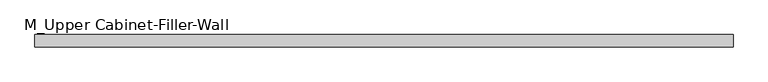
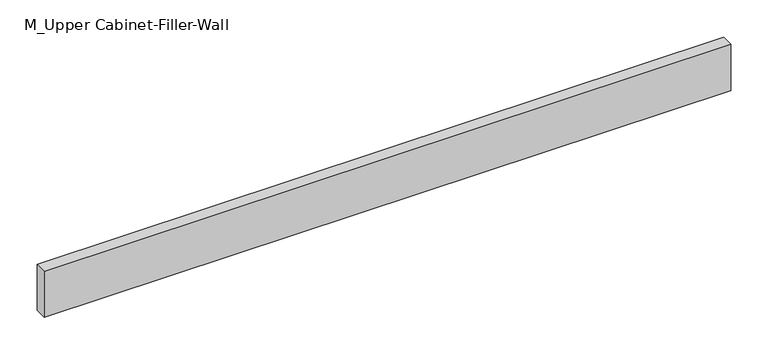
"""IFC4 building model written with IfcOpenShell, lengths in millimetres: furniture geometry, M_Upper Cabinet-Filler-Wall : fhorizontal2."""

from ifc_helpers import new_model, si_unit, frame, origin, place, context, project, spatial, polyline, outline, extrude, source, transform, mapped, element, save


def m_upper_cabinet_filler_wall_ea785238(model_context):
    return source(origin(), model_context, "Body", "SweptSolid", [
        extrude(outline(polyline([(-503.6288372, 38.1), (-503.6288372, 57.15), (563.1711628, 57.15), (563.1711628, 38.1), (-503.6288372, 38.1)])), frame((0.0, 0.0, 1923.8), z_axis=(0.0, 0.0, 1.0), x_axis=(1.0, 0.0, 0.0)), (0.0, 0.0, 1.0), 76.2),
    ])


if __name__ == "__main__":
    model = new_model("IFC4")
    model_context = context("Model", 3, world=origin())
    ifc_project = project(units=[si_unit("LENGTHUNIT", "METRE", prefix="MILLI")], contexts=[model_context])
    site = spatial("IfcSite", under=ifc_project)
    building = spatial("IfcBuilding", under=site)
    placement = place(None, origin())
    m_upper_cabinet_filler_wall_shape = m_upper_cabinet_filler_wall_ea785238(model_context)
    element("IfcFurniture", 1, ObjectType="M_Upper Cabinet-Filler-Wall : fhorizontal2", at=placement, inside=building, context=model_context, shape_type="MappedRepresentation", body=[
        mapped(m_upper_cabinet_filler_wall_shape, transform((0.0, 0.0, 0.0), x_axis=(1.0, 0.0, 0.0), y_axis=(0.0, 1.0, 0.0), z_axis=(0.0, 0.0, 1.0))),
    ])
    save(model, "model.ifc")

# Revit data of these elements
# Type "M_Upper Cabinet-Filler-Wall : fhorizontal2"
#   Depth = 0' - 1"
#   Height = 0' - 3"
#   Top Of Cabinet = 6' - 6.74016"
#   Width = 3' - 6"
#   Cabinet Material = none
#   Default Elevation = 0
# Element 1 (IfcFurniture, "M_Upper Cabinet-Filler-Wall : fhorizontal2")
#   Materials on its faces: "Cabinets"
# Materials
#   "Cabinets": class "Miscellaneous", colour RGB 249 249 249, transparency 0
